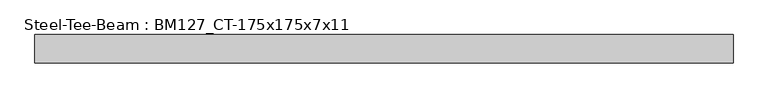
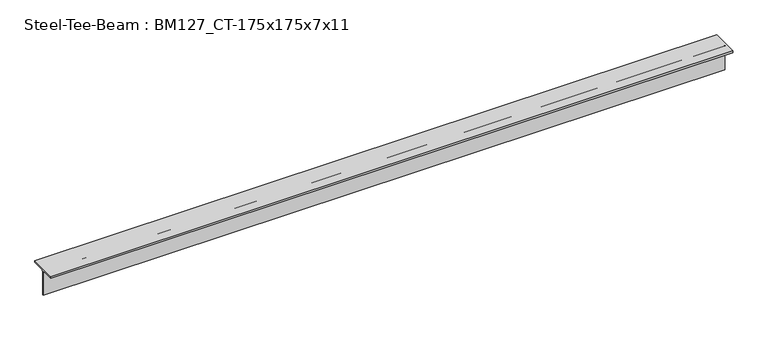
"""IFC4 building model written with IfcOpenShell, lengths in millimetres: beam geometry, Steel-Tee-Beam : BM127_CT-175x175x7x11."""

import ifcopenshell
import ifcopenshell.guid

model = None  # the IFC model being written
_history = None  # IfcOwnerHistory: only IFC2X3 demands one
_inside = {}  # id of a spatial element -> (the spatial element, [elements in it])
_under = {}  # id of a project, library or spatial element -> (it, [spatial elements below it])
_declared = {}  # id of a project -> (the project, [libraries it declares])
_typed = {}  # id of a type object -> (the type object, [elements of that type])
_made_of = {}  # id of a material, layer set ... -> (it, [elements and type objects made of it])


def new_model(schema):
    """Start an empty IFC model of exactly this schema.

    Asked for "IFC4X3", IfcOpenShell would pick the latest addendum, in which some entities
    have other attributes; the version numbers below select the first issue.
    IFC2X3 requires an IfcOwnerHistory on every rooted entity: one is made here for all.
    """
    global model, _history
    if schema == "IFC4X3":
        model = ifcopenshell.file(schema_version=(4, 3, 0, 0))
    else:
        model = ifcopenshell.file(schema=schema)
    _inside.clear()
    _under.clear()
    _declared.clear()
    _typed.clear()
    _made_of.clear()
    _history = None
    if model.schema == "IFC2X3":
        org = make("IfcOrganization", Name="unknown")
        user = make(
            "IfcPersonAndOrganization",
            ThePerson=make("IfcPerson", FamilyName="unknown"),
            TheOrganization=org,
        )
        app = make(
            "IfcApplication",
            ApplicationDeveloper=org,
            Version="unknown",
            ApplicationFullName="unknown",
            ApplicationIdentifier="unknown",
        )
        _history = make(
            "IfcOwnerHistory",
            OwningUser=user,
            OwningApplication=app,
            ChangeAction="ADDED",
            CreationDate=0,
        )
    return model


def make(cls, **values):
    """One entity of the class cls with the attributes given. An attribute that is None is left unset."""
    return model.create_entity(
        cls, **{name: value for name, value in values.items() if value is not None}
    )


def rooted(cls, **values):
    """An entity with a GlobalId (a new one), such as an element, a storey or a relation."""
    return make(cls, GlobalId=ifcopenshell.guid.new(), OwnerHistory=_history, **values)


def si_unit(unit_type, name, prefix=None):
    """IfcSIUnit, for example si_unit("LENGTHUNIT", "METRE", prefix="MILLI")."""
    return make("IfcSIUnit", UnitType=unit_type, Prefix=prefix, Name=name)


def assignment(units):
    """IfcUnitAssignment: the units of a project."""
    return None if units is None else make("IfcUnitAssignment", Units=units)


def point(xyz):
    """IfcCartesianPoint."""
    return None if xyz is None else make("IfcCartesianPoint", Coordinates=xyz)


def direction(xyz):
    """IfcDirection."""
    return None if xyz is None else make("IfcDirection", DirectionRatios=xyz)


def frame(location, z_axis=None, x_axis=None):
    """IfcAxis2Placement3D, a coordinate frame: its origin and axes. An axis left out is left unset."""
    return make(
        "IfcAxis2Placement3D",
        Location=point(location),
        Axis=direction(z_axis),
        RefDirection=direction(x_axis),
    )


def frame_2d(location, x_axis=None):
    """IfcAxis2Placement2D, a coordinate frame in the plane: its origin and x axis."""
    return make(
        "IfcAxis2Placement2D", Location=point(location), RefDirection=direction(x_axis)
    )


def origin():
    """The frame at (0, 0, 0) with its axes left unset."""
    return frame((0.0, 0.0, 0.0))


def place(relative_to, where):
    """IfcLocalPlacement: puts the frame where relative to a parent placement (None: the world)."""
    return make(
        "IfcLocalPlacement", PlacementRelTo=relative_to, RelativePlacement=where
    )


def context(
    kind, dimensions, precision=None, world=None, true_north=None, identifier=None
):
    """IfcGeometricRepresentationContext, for example the 3D "Model" context."""
    return make(
        "IfcGeometricRepresentationContext",
        ContextIdentifier=identifier,
        ContextType=kind,
        CoordinateSpaceDimension=dimensions,
        Precision=precision,
        WorldCoordinateSystem=world,
        TrueNorth=true_north,
    )


def project(units=None, contexts=None):
    """IfcProject with its units and contexts."""
    return rooted(
        "IfcProject",
        Name="project",
        RepresentationContexts=contexts,
        UnitsInContext=assignment(units),
    )


def spatial(cls, under=None, at=None, **own):
    """A site, building, storey or space (cls), placed at a placement, below another one or the project."""
    s = rooted(cls, ObjectPlacement=at, **own)
    if under is not None:
        _under.setdefault(under.id(), (under, []))[1].append(s)
    return s


def polyline(points):
    """IfcPolyline through the points."""
    return make("IfcPolyline", Points=[point(p) for p in points])


def circle_curve(where, radius):
    """IfcCircle in the frame where."""
    return make("IfcCircle", Position=where, Radius=radius)


def trimmed(basis, trim1, trim2, sense, master):
    """IfcTrimmedCurve: the piece of a basis curve between two trims."""
    return make(
        "IfcTrimmedCurve",
        BasisCurve=basis,
        Trim1=trim1,
        Trim2=trim2,
        SenseAgreement=sense,
        MasterRepresentation=master,
    )


def segment(curve, same_sense, transition):
    """IfcCompositeCurveSegment."""
    return make(
        "IfcCompositeCurveSegment",
        Transition=transition,
        SameSense=same_sense,
        ParentCurve=curve,
    )


def composite_curve(segments, self_intersect=None):
    """IfcCompositeCurve: segments joined end to end."""
    return make("IfcCompositeCurve", Segments=segments, SelfIntersect=self_intersect)


def outline(outer, holes=None, kind="AREA"):
    """IfcArbitraryClosedProfileDef: a profile drawn as a closed curve; with holes, ...WithVoids."""
    if holes is None:
        return make("IfcArbitraryClosedProfileDef", ProfileType=kind, OuterCurve=outer)
    return make(
        "IfcArbitraryProfileDefWithVoids",
        ProfileType=kind,
        OuterCurve=outer,
        InnerCurves=holes,
    )


def extrude(swept, where, along, depth):
    """IfcExtrudedAreaSolid: the profile swept, set in the frame where, extruded along a direction by depth."""
    return make(
        "IfcExtrudedAreaSolid",
        SweptArea=swept,
        Position=where,
        ExtrudedDirection=direction(along),
        Depth=depth,
    )


def shape(context_of_items, identifier, shape_type, items):
    """IfcShapeRepresentation: the items that make up one representation, for example the "Body"."""
    return make(
        "IfcShapeRepresentation",
        ContextOfItems=context_of_items,
        RepresentationIdentifier=identifier,
        RepresentationType=shape_type,
        Items=items,
    )


def source(mapping_origin, context_of_items, identifier, shape_type, items):
    """IfcRepresentationMap: a shape defined once, which mapped items show again and again."""
    return make(
        "IfcRepresentationMap",
        MappingOrigin=mapping_origin,
        MappedRepresentation=shape(context_of_items, identifier, shape_type, items),
    )


def transform(
    local_origin,
    x_axis=None,
    y_axis=None,
    z_axis=None,
    scale=None,
    scale2=None,
    scale3=None,
    uniform=True,
):
    """IfcCartesianTransformationOperator3D, or its non-uniform kind. x_axis, y_axis, z_axis: its Axis1, 2, 3."""
    if uniform:
        return make(
            "IfcCartesianTransformationOperator3D",
            Axis1=direction(x_axis),
            Axis2=direction(y_axis),
            LocalOrigin=point(local_origin),
            Scale=scale,
            Axis3=direction(z_axis),
        )
    return make(
        "IfcCartesianTransformationOperator3DnonUniform",
        Axis1=direction(x_axis),
        Axis2=direction(y_axis),
        LocalOrigin=point(local_origin),
        Scale=scale,
        Axis3=direction(z_axis),
        Scale2=scale2,
        Scale3=scale3,
    )


def mapped(mapping_source, mapping_target):
    """IfcMappedItem: shows the shape of a source again, moved by a transform."""
    return make(
        "IfcMappedItem", MappingSource=mapping_source, MappingTarget=mapping_target
    )


def made_of(thing, what):
    """Note that an element or type object is made of a material, layer set ...; save() writes the relation."""
    if what is not None:
        _made_of.setdefault(what.id(), (what, []))[1].append(thing)
    return thing


def element(
    cls,
    number,
    at=None,
    inside=None,
    cuts=None,
    type_object=None,
    material=None,
    context=None,
    identifier="Body",
    shape_type=None,
    held_by="IfcProductDefinitionShape",
    body=None,
    shapes=None,
    **own,
):
    """One element of the class cls, such as IfcWall. Its Tag is "e" and its number.

    at: its placement. inside: the storey or other place that contains it. cuts: it is an
    opening in that element (IfcRelVoidsElement). A single representation is given by context,
    identifier, shape_type and body (its items); several are given by shapes. held_by: the class
    of the entity that holds the representations. save() writes the other relations.
    """
    e = rooted(cls, Tag="e%d" % number, ObjectPlacement=at, **own)
    if body is not None:
        shapes = [shape(context, identifier, shape_type, body)]
    if shapes is not None:
        e.Representation = make(held_by, Representations=shapes)
    if inside is not None:
        _inside.setdefault(inside.id(), (inside, []))[1].append(e)
    if cuts is not None:
        rooted(
            "IfcRelVoidsElement", RelatingBuildingElement=cuts, RelatedOpeningElement=e
        )
    if type_object is not None:
        _typed.setdefault(type_object.id(), (type_object, []))[1].append(e)
    return made_of(e, material)


def aggregate(whole, parts):
    """IfcRelAggregates: a whole, such as a stair, and the parts it consists of."""
    return rooted("IfcRelAggregates", RelatingObject=whole, RelatedObjects=parts)


def save(model, path):
    """Write the relations noted so far, then the file.

    IfcRelAggregates (storeys below a building ...), IfcRelContainedInSpatialStructure (elements
    in a storey), IfcRelDefinesByType, IfcRelAssociatesMaterial and IfcRelDeclares: one each for
    every whole, place, type object, material and project.
    """
    for whole, parts in _under.values():
        aggregate(whole, parts)
    for where, things in _inside.values():
        rooted(
            "IfcRelContainedInSpatialStructure",
            RelatedElements=things,
            RelatingStructure=where,
        )
    for kind, things in _typed.values():
        rooted("IfcRelDefinesByType", RelatedObjects=things, RelatingType=kind)
    for what, things in _made_of.values():
        rooted("IfcRelAssociatesMaterial", RelatedObjects=things, RelatingMaterial=what)
    for by, libraries in _declared.values():
        rooted("IfcRelDeclares", RelatingContext=by, RelatedDefinitions=libraries)
    model.write(path)


def steel_tee_beam_bm127_ct_175x175x7x11_5181b933(model_context):
    return source(origin(), model_context, "Body", "SweptSolid", [
        extrude(outline(composite_curve([segment(polyline([(87.5, 87.5), (87.5, 76.5), (17.5, 76.5)]), True, "CONTINUOUS"), segment(trimmed(circle_curve(frame_2d((17.5, 62.5)), 14.0), [point((17.5, 76.5))], [point((3.5, 62.5))], True, "CARTESIAN"), True, "CONTINUOUS"), segment(polyline([(3.5, 62.5), (3.5, -87.5), (-3.5, -87.5), (-3.5, 62.5)]), True, "CONTINUOUS"), segment(trimmed(circle_curve(frame_2d((-17.5, 62.5)), 14.0), [point((-3.5, 62.5))], [point((-17.5, 76.5))], True, "CARTESIAN"), True, "CONTINUOUS"), segment(polyline([(-17.5, 76.5), (-87.5, 76.5), (-87.5, 87.5), (87.5, 87.5)]), True, "CONTINUOUS")], self_intersect=False)), frame((-2106.825064, 0.0, 0.0), z_axis=(1.0, 0.0, 0.0), x_axis=(0.0, 1.0, 0.0)), (0.0, 0.0, 1.0), 4291.0318249),
    ])


if __name__ == "__main__":
    model = new_model("IFC4")
    model_context = context("Model", 3, world=origin())
    ifc_project = project(units=[si_unit("LENGTHUNIT", "METRE", prefix="MILLI")], contexts=[model_context])
    site = spatial("IfcSite", under=ifc_project)
    building = spatial("IfcBuilding", under=site)
    placement = place(None, origin())
    steel_tee_beam_bm127_ct_175x175x7x11_shape = steel_tee_beam_bm127_ct_175x175x7x11_5181b933(model_context)
    element("IfcBeam", 1, ObjectType="Steel-Tee-Beam : BM127_CT-175x175x7x11", at=placement, inside=building, context=model_context, shape_type="MappedRepresentation", body=[
        mapped(steel_tee_beam_bm127_ct_175x175x7x11_shape, transform((0.0, 0.0, 0.0), x_axis=(1.0, 0.0, 0.0), y_axis=(0.0, 1.0, 0.0), z_axis=(0.0, 0.0, 1.0))),
    ])
    save(model, "model.ifc")

# Revit data of these elements
# Type "Steel-Tee-Beam : BM127_CT-175x175x7x11"
#   Section Area = 31.57 cm²
#   Mass per Unit Length = 24.80 kg/m
#   Length [instance default] = 1524 mm
#   bf = 175 mm
#   d = 175 mm
#   k = 25 mm
#   kr = 14 mm
#   tf = 11 mm
#   tw = 7 mm
#   hec_material4 [instance default] = none
#   hec_material3 [instance default] = none
#   hec_material2 [instance default] = none
#   hec_material1 [instance default] = none
#   Structural Material [instance default] = Steel, 45-345
#   Assembly Code = ""
# Element 1 (IfcBeam, "Steel-Tee-Beam : BM127_CT-175x175x7x11")
#   hec_material3 = F01AC000-00002_Building/Shelter Fire Proofing Work_Intumescent Coating Type_1 hr. rating (UL 1709))
#   hec_material1 = S03AA029-00001_Main Steel Structure Erection Work_Shelter/Building_Light Steel
#   Structural Material = S01AA003-00001_Main Steel Structure Fabrication Work_Shelter/Building_Light Steel - Standard
#   Materials on its faces: "S01AA003-00001_Main Steel Structure Fabrication Work_Shelter/Building_Light Steel - Standard"
# Materials
#   "Steel, 45-345": class "Metal", colour RGB 189 187 185, transparency 0, Description = "Steel 345 MPa", Cost = 0
#   "S01AA003-00001_Main Steel Structure Fabrication Work_Shelter/Building_Light Steel - Standard": class "Metal", colour RGB 120 120 120, transparency 0, Comments = "(30KG/M>Weight)", Description = "Structural steel 50ksi", W00) Work Master Code = "S01AA003-00001", W01) Work Master_Lv1 = "Main Steel Structure Fabrication Work", W02) Work Master_Lv2 = "Shelter/Building", W03) Work Master_Spec.1 = "Light Steel - Standard (30KG/M>Weight)", Cost = 0
#   "F01AC000-00002_Building/Shelter Fire Proofing Work_Intumescent Coating Type_1 hr. rating (UL 1709))": class "Metal", colour RGB 255 128 128, transparency 0, Description = "Paint finished steel", W00) Work Master Code = "F01AC000-00002", W01) Work Master_Lv1 = "Building/Shelter Fire Proofing Work", W02) Work Master_Lv2 = "Intumescent Coating Type", W03) Work Master_Spec.1 = "1 hr. rating (UL 1709)", Cost = 0
#   "S03AA029-00001_Main Steel Structure Erection Work_Shelter/Building_Light Steel": class "Metal", colour RGB 120 120 120, transparency 0, Comments = "(30KG/M>Weight)", Description = "Structural steel 50ksi", W00) Work Master Code = "S03AA029-00001", W01) Work Master_Lv1 = "Main Steel Structure Erection Work", W02) Work Master_Lv2 = "Shelter/Building", W03) Work Master_Spec.1 = "Light Steel (30KG/M>Weight)", Cost = 0
